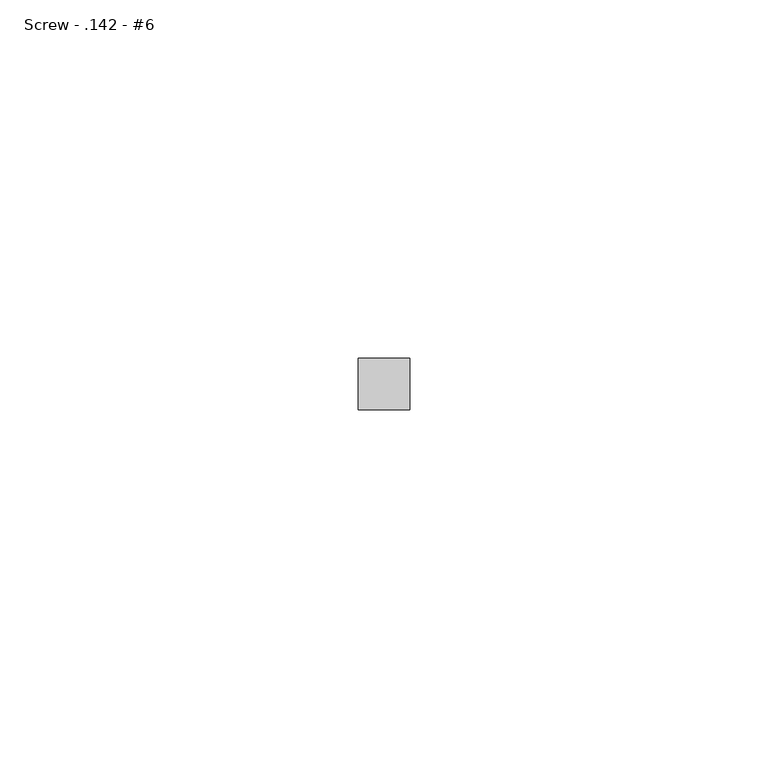
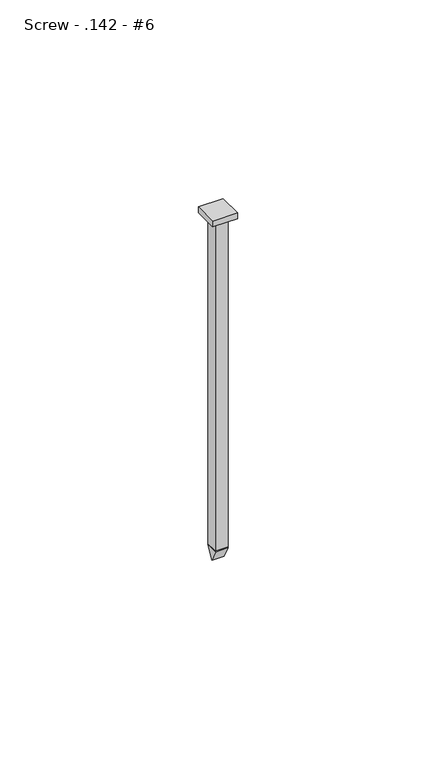
"""IFC4 building model written with IfcOpenShell, lengths in millimetres: fastener geometry, 060523 - W_P_C - Fastenings - Generic - SQUARE : Screw - .142 - #6."""

from ifc_helpers import new_model, si_unit, frame, origin, origin_with_axes, place, context, project, spatial, polyline, outline, extrude, source, transform, mapped, element, save


def screw_142_6_19bc7189(model_context):
    return source(origin(), model_context, "Body", "SweptSolid", [
        extrude(outline(polyline([(0.0, -105.2068), (-1.8034, -101.6), (1.8034, -101.6), (0.0, -105.2068)])), frame((-1.8034, 0.0, 0.0), z_axis=(1.0, 0.0, 0.0), x_axis=(0.0, 1.0, 0.0)), (0.0, 0.0, 1.0), 3.6068),
        extrude(outline(polyline([(-3.6068, -3.6068), (-3.6068, 3.6068), (3.6068, 3.6068), (3.6068, -3.6068), (-3.6068, -3.6068)])), origin_with_axes(), (0.0, 0.0, 1.0), 1.8034),
        extrude(outline(polyline([(-1.8034, 1.8034), (1.8034, 1.8034), (1.8034, -1.8034), (-1.8034, -1.8034), (-1.8034, 1.8034)])), frame((0.0, 0.0, -101.6), z_axis=(0.0, 0.0, 1.0), x_axis=(1.0, 0.0, 0.0)), (0.0, 0.0, 1.0), 101.6),
    ])


if __name__ == "__main__":
    model = new_model("IFC4")
    model_context = context("Model", 3, world=origin())
    ifc_project = project(units=[si_unit("LENGTHUNIT", "METRE", prefix="MILLI")], contexts=[model_context])
    site = spatial("IfcSite", under=ifc_project)
    building = spatial("IfcBuilding", under=site)
    placement = place(None, origin())
    screw_142_6_shape = screw_142_6_19bc7189(model_context)
    element("IfcFastener", 1, ObjectType="060523 - W_P_C - Fastenings - Generic - SQUARE : Screw - .142 - #6", at=placement, inside=building, context=model_context, shape_type="MappedRepresentation", body=[
        mapped(screw_142_6_shape, transform((0.0, 0.0, 0.0), x_axis=(1.0, 0.0, 0.0), y_axis=(0.0, 1.0, 0.0), z_axis=(0.0, 0.0, 1.0))),
    ])
    save(model, "model.ifc")

# Revit data of these elements
# Type "060523 - W_P_C - Fastenings - Generic - SQUARE : Screw - .142 - #6"
#   Washer_Thickness = 0' - 0.00333"
#   Washer Radius = 0' - 0.081"
#   Washer Offset - Head = 0' - 0"
#   Washer Offset = 0' - 0"
#   Thickness_of_Substrate [instance default] = 0' - 1"
#   Side = 0' - 0 37/64"
#   Radius = 0' - 0.071"
#   Length [instance default] = 0' - 4"
#   Head Size = 0' - 1"
#   Head Radius = 0' - 0 1/2"
#   Head Height = 0' - 0.01"
#   Double Diameter = 0' - 0.284"
#   Diameter = 0' - 0.142"
#   Default Elevation = 4' - 0"
#   Washer_Nut_Visibility = no
#   Washer_Head_Visibility = no
#   Round_Head_Visibility = yes
#   Point Visibility = yes
#   Nut_Visibility = no
#   Hex_Head_Visiblilty = no
#   Washer Material = none
#   Bolt Material (Size) = AT SILL - FASTENER AT 24" O.C.
# Materials
#   "AT SILL - FASTENER AT 24\" O.C.": class "Generic", colour RGB 120 120 120, transparency 0, Cost = 0
